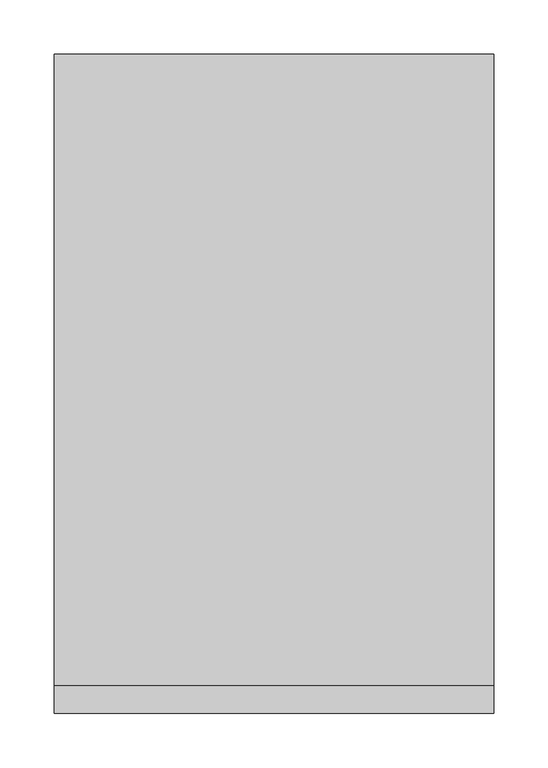
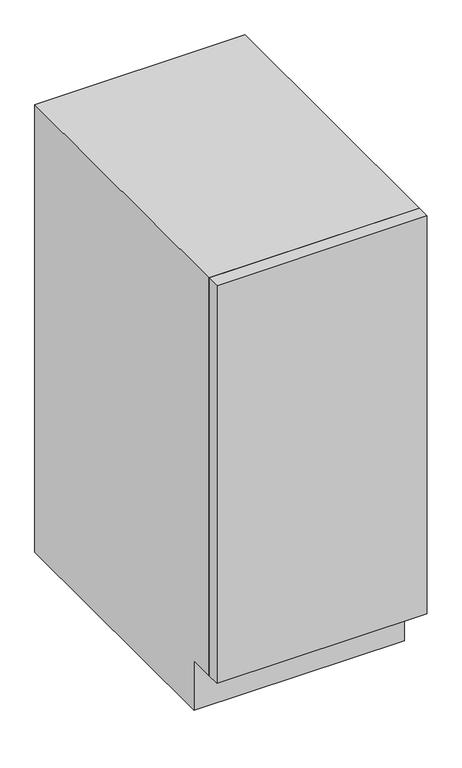
"""IFC4 building model written with IfcOpenShell, lengths in millimetres: furniture geometry, OD_CW_Base Cabinet : OD_CW_Base Cabinet."""

from ifc_helpers import new_model, si_unit, frame, origin, place, context, project, spatial, polyline, outline, extrude, source, transform, mapped, element, save


def furniture_054c2b87(model_context):
    return source(origin(), model_context, "Body", "SweptSolid", [
        extrude(outline(polyline([(18.7377049, 25.4), (425.1377049, 25.4), (425.1377049, 0.0), (18.7377049, 0.0), (18.7377049, 25.4)])), frame((0.0, 0.0, 101.6), z_axis=(0.0, 0.0, 1.0), x_axis=(1.0, 0.0, 0.0)), (0.0, 0.0, 1.0), 812.8),
        extrude(outline(polyline([(25.4, 914.4), (609.6, 914.4), (609.6, 0.0), (76.2, 0.0), (76.2, 101.6), (25.4, 101.6), (25.4, 914.4)])), frame((18.7377049, 0.0, 0.0), z_axis=(1.0, 0.0, 0.0), x_axis=(0.0, 1.0, 0.0)), (0.0, 0.0, 1.0), 406.4),
    ])


if __name__ == "__main__":
    model = new_model("IFC4")
    model_context = context("Model", 3, world=origin())
    ifc_project = project(units=[si_unit("LENGTHUNIT", "METRE", prefix="MILLI")], contexts=[model_context])
    site = spatial("IfcSite", under=ifc_project)
    building = spatial("IfcBuilding", under=site)
    placement = place(None, origin())
    furniture_shape = furniture_054c2b87(model_context)
    element("IfcFurniture", 1, ObjectType="OD_CW_Base Cabinet : OD_CW_Base Cabinet", at=placement, inside=building, context=model_context, shape_type="MappedRepresentation", body=[
        mapped(furniture_shape, transform((0.0, 0.0, 0.0), x_axis=(1.0, 0.0, 0.0), y_axis=(0.0, 1.0, 0.0), z_axis=(0.0, 0.0, 1.0))),
    ])
    save(model, "model.ifc")

# Revit data of these elements
# Type "OD_CW_Base Cabinet : OD_CW_Base Cabinet"
#   OD_CW_Width [instance default] = 2' - 10"
#   OD_CW_Length [instance default] = 8' - 0"
#   OD_CW_Height [instance default] = 2' - 3"
#   Depth = 2' - 0"
#   Height = 3' - 0"
#   Width = 4' - 0"
#   OD_CW_Material_Front Panel [instance default] = none
#   OD_CW_Material_Body [instance default] = none
# Element 1 (IfcFurniture, "OD_CW_Base Cabinet : OD_CW_Base Cabinet")
#   OD_CW_Width = 2' - 0"
#   OD_CW_Length = 1' - 4"
#   OD_CW_Height = 3' - 0"
#   OD_CW_Material_Body = DOUGH TRAY
#   Materials on its faces: "DOUGH TRAY", "CASEWORK"
# Materials
#   "DOUGH TRAY": class "Generic", colour RGB 187 187 187, transparency 0, Cost = 0
#   "CASEWORK": class "Generic", colour RGB 181 181 181, transparency 0, Cost = 0
